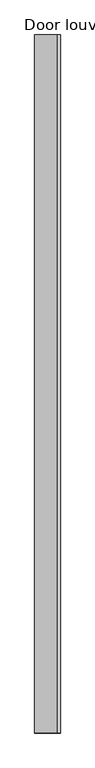
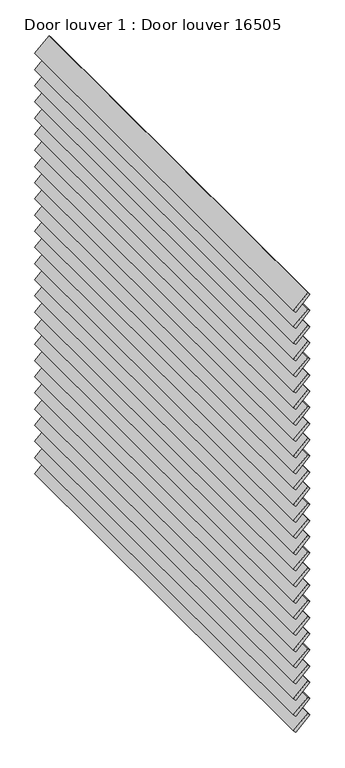
"""IFC4 building model written with IfcOpenShell, lengths in millimetres: proxy geometry, Door louver 1 : Door louver 16505."""

from ifc_helpers import new_model, si_unit, frame, origin, place, context, project, spatial, polyline, outline, extrude, source, transform, mapped, element, save


def door_louver_1_door_louver_16505_7676acec(model_context):
    return source(origin(), model_context, "Body", "SweptSolid", [
        extrude(outline(polyline([(0.0, -88.6), (0.0, 0.0), (2000.0, 0.0), (2000.0, -88.6), (0.0, -88.6)])), frame((-8304.3306423, 6540.4513244, 32854.8547367), z_axis=(-0.6925092278135618, 0.0, 0.721409016711785), x_axis=(0.0, -1.0, 0.0)), (0.0, 0.0, 1.0), 13.8216714),
        extrude(outline(polyline([(0.0, -88.6), (0.0, 0.0), (2000.0, 0.0), (2000.0, -88.6), (0.0, -88.6)])), frame((-8304.3306423, 6540.4513244, 32931.0547367), z_axis=(-0.6925092278135618, 0.0, 0.721409016711785), x_axis=(0.0, -1.0, 0.0)), (0.0, 0.0, 1.0), 13.8216714),
        extrude(outline(polyline([(0.0, -88.6), (0.0, 0.0), (2000.0, 0.0), (2000.0, -88.6), (0.0, -88.6)])), frame((-8304.3306423, 6540.4513244, 33007.2547367), z_axis=(-0.6925092278135618, 0.0, 0.721409016711785), x_axis=(0.0, -1.0, 0.0)), (0.0, 0.0, 1.0), 13.8216714),
        extrude(outline(polyline([(0.0, -88.6), (0.0, 0.0), (2000.0, 0.0), (2000.0, -88.6), (0.0, -88.6)])), frame((-8304.3306423, 6540.4513244, 33083.4547367), z_axis=(-0.6925092278135618, 0.0, 0.721409016711785), x_axis=(0.0, -1.0, 0.0)), (0.0, 0.0, 1.0), 13.8216714),
        extrude(outline(polyline([(0.0, -88.6), (0.0, 0.0), (2000.0, 0.0), (2000.0, -88.6), (0.0, -88.6)])), frame((-8304.3306423, 6540.4513244, 33159.6547367), z_axis=(-0.6925092278135618, 0.0, 0.721409016711785), x_axis=(0.0, -1.0, 0.0)), (0.0, 0.0, 1.0), 13.8216714),
        extrude(outline(polyline([(0.0, -88.6), (0.0, 0.0), (2000.0, 0.0), (2000.0, -88.6), (0.0, -88.6)])), frame((-8304.3306423, 6540.4513244, 33235.8547367), z_axis=(-0.6925092278135618, 0.0, 0.721409016711785), x_axis=(0.0, -1.0, 0.0)), (0.0, 0.0, 1.0), 13.8216714),
        extrude(outline(polyline([(0.0, -88.6), (0.0, 0.0), (2000.0, 0.0), (2000.0, -88.6), (0.0, -88.6)])), frame((-8304.3306423, 6540.4513244, 33312.0547367), z_axis=(-0.6925092278135618, 0.0, 0.721409016711785), x_axis=(0.0, -1.0, 0.0)), (0.0, 0.0, 1.0), 13.8216714),
        extrude(outline(polyline([(0.0, -88.6), (0.0, 0.0), (2000.0, 0.0), (2000.0, -88.6), (0.0, -88.6)])), frame((-8304.3306423, 6540.4513244, 33388.2547367), z_axis=(-0.6925092278135618, 0.0, 0.721409016711785), x_axis=(0.0, -1.0, 0.0)), (0.0, 0.0, 1.0), 13.8216714),
        extrude(outline(polyline([(0.0, -88.6), (0.0, 0.0), (2000.0, 0.0), (2000.0, -88.6), (0.0, -88.6)])), frame((-8304.3306423, 6540.4513244, 33464.4547367), z_axis=(-0.6925092278135618, 0.0, 0.721409016711785), x_axis=(0.0, -1.0, 0.0)), (0.0, 0.0, 1.0), 13.8216714),
        extrude(outline(polyline([(0.0, -88.6), (0.0, 0.0), (2000.0, 0.0), (2000.0, -88.6), (0.0, -88.6)])), frame((-8304.3306423, 6540.4513244, 33540.6547367), z_axis=(-0.6925092278135618, 0.0, 0.721409016711785), x_axis=(0.0, -1.0, 0.0)), (0.0, 0.0, 1.0), 13.8216714),
        extrude(outline(polyline([(0.0, -88.6), (0.0, 0.0), (2000.0, 0.0), (2000.0, -88.6), (0.0, -88.6)])), frame((-8304.3306423, 6540.4513244, 33616.8547367), z_axis=(-0.6925092278135618, 0.0, 0.721409016711785), x_axis=(0.0, -1.0, 0.0)), (0.0, 0.0, 1.0), 13.8216714),
        extrude(outline(polyline([(0.0, -88.6), (0.0, 0.0), (2000.0, 0.0), (2000.0, -88.6), (0.0, -88.6)])), frame((-8304.3306423, 6540.4513244, 33693.0547367), z_axis=(-0.6925092278135618, 0.0, 0.721409016711785), x_axis=(0.0, -1.0, 0.0)), (0.0, 0.0, 1.0), 13.8216714),
        extrude(outline(polyline([(0.0, -88.6), (0.0, 0.0), (2000.0, 0.0), (2000.0, -88.6), (0.0, -88.6)])), frame((-8304.3306423, 6540.4513244, 33769.2547367), z_axis=(-0.6925092278135618, 0.0, 0.721409016711785), x_axis=(0.0, -1.0, 0.0)), (0.0, 0.0, 1.0), 13.8216714),
        extrude(outline(polyline([(0.0, -88.6), (0.0, 0.0), (2000.0, 0.0), (2000.0, -88.6), (0.0, -88.6)])), frame((-8304.3306423, 6540.4513244, 33845.4547367), z_axis=(-0.6925092278135618, 0.0, 0.721409016711785), x_axis=(0.0, -1.0, 0.0)), (0.0, 0.0, 1.0), 13.8216714),
        extrude(outline(polyline([(0.0, -88.6), (0.0, 0.0), (2000.0, 0.0), (2000.0, -88.6), (0.0, -88.6)])), frame((-8304.3306423, 6540.4513244, 33921.6547367), z_axis=(-0.6925092278135618, 0.0, 0.721409016711785), x_axis=(0.0, -1.0, 0.0)), (0.0, 0.0, 1.0), 13.8216714),
        extrude(outline(polyline([(0.0, -88.6), (0.0, 0.0), (2000.0, 0.0), (2000.0, -88.6), (0.0, -88.6)])), frame((-8304.3306423, 6540.4513244, 33997.8547367), z_axis=(-0.6925092278135618, 0.0, 0.721409016711785), x_axis=(0.0, -1.0, 0.0)), (0.0, 0.0, 1.0), 13.8216714),
        extrude(outline(polyline([(0.0, -88.6), (0.0, 0.0), (2000.0, 0.0), (2000.0, -88.6), (0.0, -88.6)])), frame((-8304.3306423, 6540.4513244, 34074.0547367), z_axis=(-0.6925092278135618, 0.0, 0.721409016711785), x_axis=(0.0, -1.0, 0.0)), (0.0, 0.0, 1.0), 13.8216714),
        extrude(outline(polyline([(0.0, -88.6), (0.0, 0.0), (2000.0, 0.0), (2000.0, -88.6), (0.0, -88.6)])), frame((-8304.3306423, 6540.4513244, 34150.2547367), z_axis=(-0.6925092278135618, 0.0, 0.721409016711785), x_axis=(0.0, -1.0, 0.0)), (0.0, 0.0, 1.0), 13.8216714),
        extrude(outline(polyline([(0.0, -88.6), (0.0, 0.0), (2000.0, 0.0), (2000.0, -88.6), (0.0, -88.6)])), frame((-8304.3306423, 6540.4513244, 34226.4547367), z_axis=(-0.6925092278135618, 0.0, 0.721409016711785), x_axis=(0.0, -1.0, 0.0)), (0.0, 0.0, 1.0), 13.8216714),
        extrude(outline(polyline([(0.0, -88.6), (0.0, 0.0), (2000.0, 0.0), (2000.0, -88.6), (0.0, -88.6)])), frame((-8304.3306423, 6540.4513244, 34302.6547367), z_axis=(-0.6925092278135618, 0.0, 0.721409016711785), x_axis=(0.0, -1.0, 0.0)), (0.0, 0.0, 1.0), 13.8216714),
        extrude(outline(polyline([(0.0, -88.6), (0.0, 0.0), (2000.0, 0.0), (2000.0, -88.6), (0.0, -88.6)])), frame((-8304.3306423, 6540.4513244, 34378.8547367), z_axis=(-0.6925092278135618, 0.0, 0.721409016711785), x_axis=(0.0, -1.0, 0.0)), (0.0, 0.0, 1.0), 13.8216714),
        extrude(outline(polyline([(0.0, -88.6), (0.0, 0.0), (2000.0, 0.0), (2000.0, -88.6), (0.0, -88.6)])), frame((-8304.3306423, 6540.4513244, 34455.0547367), z_axis=(-0.6925092278135618, 0.0, 0.721409016711785), x_axis=(0.0, -1.0, 0.0)), (0.0, 0.0, 1.0), 13.8216714),
        extrude(outline(polyline([(0.0, -88.6), (0.0, 0.0), (2000.0, 0.0), (2000.0, -88.6), (0.0, -88.6)])), frame((-8304.3306423, 6540.4513244, 34531.2547367), z_axis=(-0.6925092278135618, 0.0, 0.721409016711785), x_axis=(0.0, -1.0, 0.0)), (0.0, 0.0, 1.0), 13.8216714),
        extrude(outline(polyline([(0.0, -88.6), (0.0, 0.0), (2000.0, 0.0), (2000.0, -88.6), (0.0, -88.6)])), frame((-8304.3306423, 6540.4513244, 34607.4547367), z_axis=(-0.6925092278135618, 0.0, 0.721409016711785), x_axis=(0.0, -1.0, 0.0)), (0.0, 0.0, 1.0), 13.8216714),
        extrude(outline(polyline([(0.0, -88.6), (0.0, 0.0), (2000.0, 0.0), (2000.0, -88.6), (0.0, -88.6)])), frame((-8304.3306423, 6540.4513244, 34683.6547367), z_axis=(-0.6925092278135618, 0.0, 0.721409016711785), x_axis=(0.0, -1.0, 0.0)), (0.0, 0.0, 1.0), 13.8216714),
        extrude(outline(polyline([(0.0, -88.6), (0.0, 0.0), (2000.0, 0.0), (2000.0, -88.6), (0.0, -88.6)])), frame((-8304.3306423, 6540.4513244, 34759.8547367), z_axis=(-0.6925092278135618, 0.0, 0.721409016711785), x_axis=(0.0, -1.0, 0.0)), (0.0, 0.0, 1.0), 13.8216714),
        extrude(outline(polyline([(0.0, -88.6), (0.0, 0.0), (2000.0, 0.0), (2000.0, -88.6), (0.0, -88.6)])), frame((-8304.3306423, 6540.4513244, 34836.0547367), z_axis=(-0.6925092278135618, 0.0, 0.721409016711785), x_axis=(0.0, -1.0, 0.0)), (0.0, 0.0, 1.0), 13.8216714),
    ])


if __name__ == "__main__":
    model = new_model("IFC4")
    model_context = context("Model", 3, world=origin())
    ifc_project = project(units=[si_unit("LENGTHUNIT", "METRE", prefix="MILLI")], contexts=[model_context])
    site = spatial("IfcSite", under=ifc_project)
    building = spatial("IfcBuilding", under=site)
    placement = place(None, origin())
    door_louver_1_door_louver_16505_shape = door_louver_1_door_louver_16505_7676acec(model_context)
    element("IfcBuildingElementProxy", 1, Name="Door louver 1 : Door louver 16505", ObjectType="Door louver 1 : Door louver 16505", at=placement, inside=building, context=model_context, shape_type="MappedRepresentation", body=[
        mapped(door_louver_1_door_louver_16505_shape, transform((0.0, 0.0, 0.0), x_axis=(1.0, 0.0, 0.0), y_axis=(0.0, 1.0, 0.0), z_axis=(0.0, 0.0, 1.0))),
    ])
    save(model, "model.ifc")

# Revit data of these elements
# Type "Door louver 1 : Door louver 16505"
#   NameOverride = "Door louver"
# Element 1 (IfcBuildingElementProxy, "Door louver 1 : Door louver 16505")
#   Materials on its faces: "WOODEN LOUVERS (SPEC T. B. D.)"
# Materials
#   "WOODEN LOUVERS (SPEC T. B. D.)": class "Unassigned", colour RGB 148 103 60, transparency 0, Cost = 0
